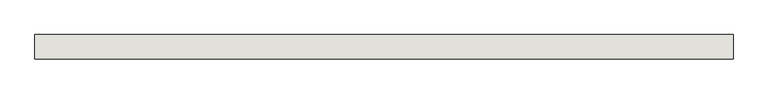
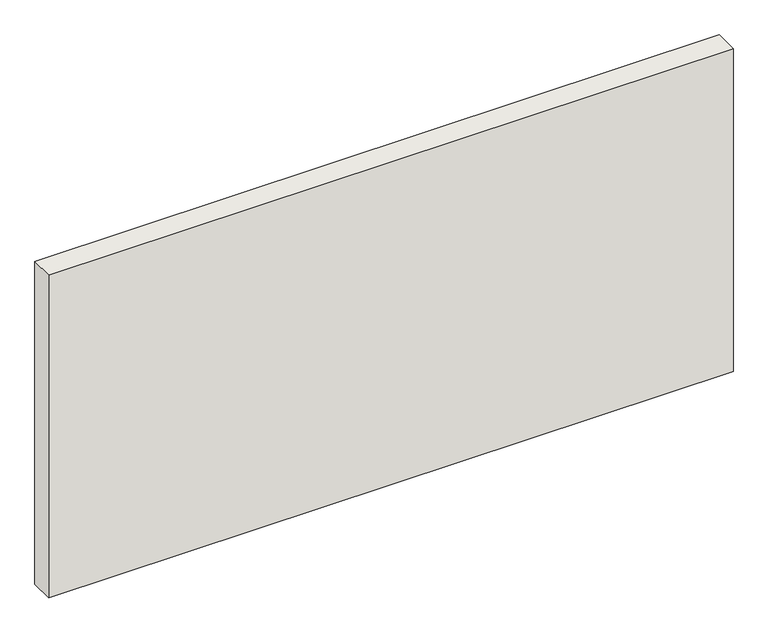
"""IFC4 building model written with IfcOpenShell, lengths in millimetres: wall geometry, Holzwand."""

from ifc_helpers import new_model, si_unit, origin, origin_with_axes, place, context, project, spatial, polyline, outline, extrude, source, transform, mapped, element, save


def wall_a479c20e(model_context):
    return source(origin(), model_context, "Body", "SweptSolid", [
        extrude(outline(polyline([(5770.0, 200.0), (5770.0, 0.0), (0.0, 0.0), (0.0, 200.0), (5770.0, 200.0)])), origin_with_axes(), (0.0, 0.0, 1.0), 2880.0),
    ])


if __name__ == "__main__":
    model = new_model("IFC4")
    model_context = context("Model", 3, world=origin())
    ifc_project = project(units=[si_unit("LENGTHUNIT", "METRE", prefix="MILLI")], contexts=[model_context])
    site = spatial("IfcSite", under=ifc_project)
    building = spatial("IfcBuilding", under=site)
    placement = place(None, origin())
    wall_shape = wall_a479c20e(model_context)
    element("IfcWall", 1, ObjectType="Holzwand", at=placement, inside=building, context=model_context, shape_type="MappedRepresentation", body=[
        mapped(wall_shape, transform((0.0, 0.0, 0.0), x_axis=(1.0, 0.0, 0.0), y_axis=(0.0, 1.0, 0.0), z_axis=(0.0, 0.0, 1.0))),
    ])
    save(model, "model.ifc")

# Revit data of these elements
# Element 1 (IfcWall, "Holzwand")
#   Materials on its faces: "holzschalung"
# Materials
#   "holzschalung": class "Unassigned", colour RGB 128 128 128, transparency 0
